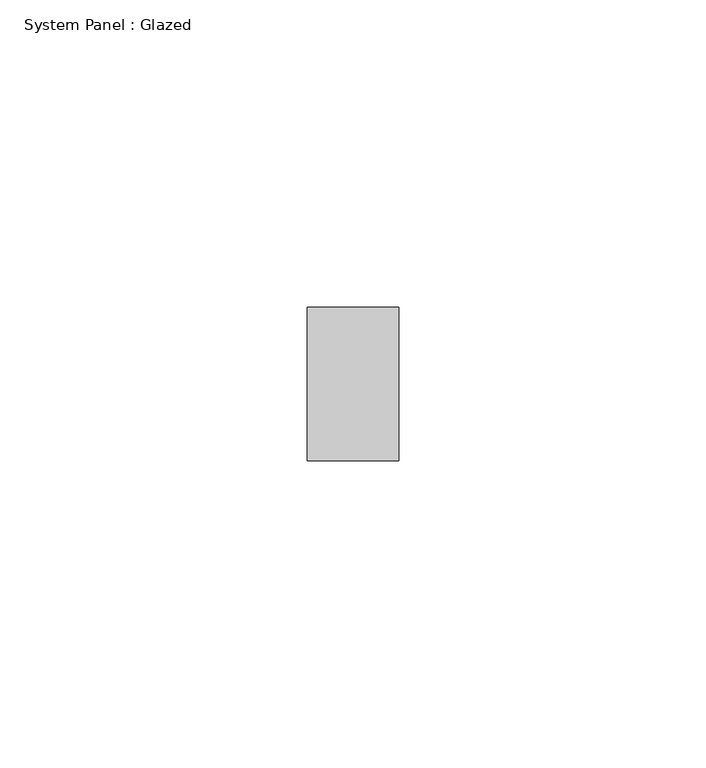
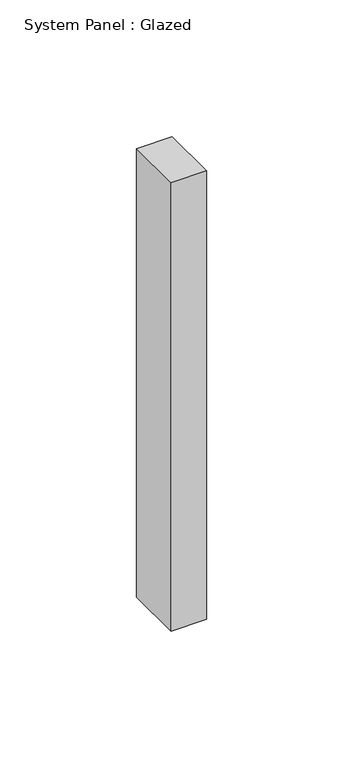
"""IFC4 building model written with IfcOpenShell, lengths in millimetres: plate geometry, System Panel : Glazed."""

from ifc_helpers import new_model, si_unit, origin, origin_with_axes, place, context, project, spatial, polyline, outline, extrude, source, transform, mapped, element, save


def system_panel_glazed_3bc540b8(model_context):
    return source(origin(), model_context, "Body", "SweptSolid", [
        extrude(outline(polyline([(7.4693035, 24.5), (-7.4693035, 24.5), (-7.4693035, 49.5), (7.4693035, 49.5), (7.4693035, 24.5)])), origin_with_axes(), (0.0, 0.0, 1.0), 200.0),
    ])


if __name__ == "__main__":
    model = new_model("IFC4")
    model_context = context("Model", 3, world=origin())
    ifc_project = project(units=[si_unit("LENGTHUNIT", "METRE", prefix="MILLI")], contexts=[model_context])
    site = spatial("IfcSite", under=ifc_project)
    building = spatial("IfcBuilding", under=site)
    placement = place(None, origin())
    system_panel_glazed_shape = system_panel_glazed_3bc540b8(model_context)
    element("IfcPlate", 1, ObjectType="System Panel : Glazed", at=placement, inside=building, context=model_context, shape_type="MappedRepresentation", body=[
        mapped(system_panel_glazed_shape, transform((0.0, 0.0, 0.0), x_axis=(1.0, 0.0, 0.0), y_axis=(0.0, 1.0, 0.0), z_axis=(0.0, 0.0, 1.0))),
    ])
    save(model, "model.ifc")

# Revit data of these elements
# Element 1 (IfcPlate, "System Panel : Glazed")
#   Materials on its faces: "Glass"
# Materials
#   "Glass": class "Glass", colour RGB 218 227 224, transparency 0.85, Description = "Soda Lime Glass", Cost = 0
